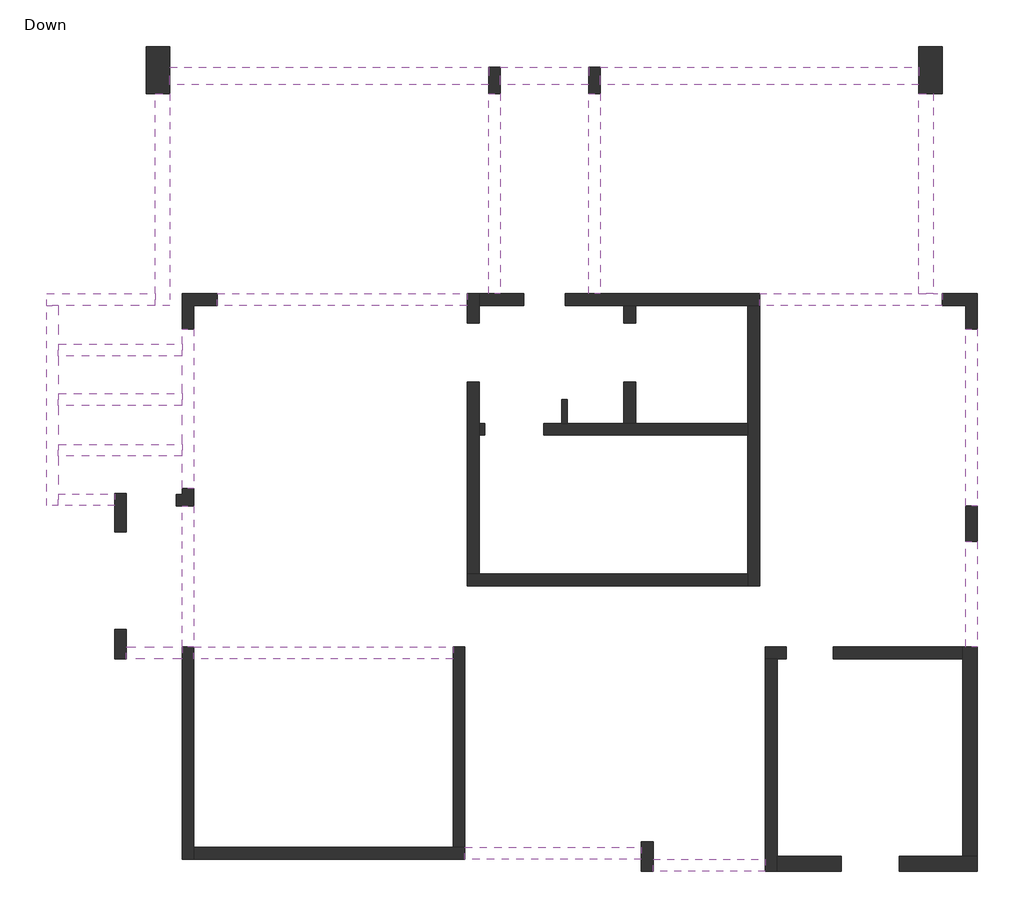
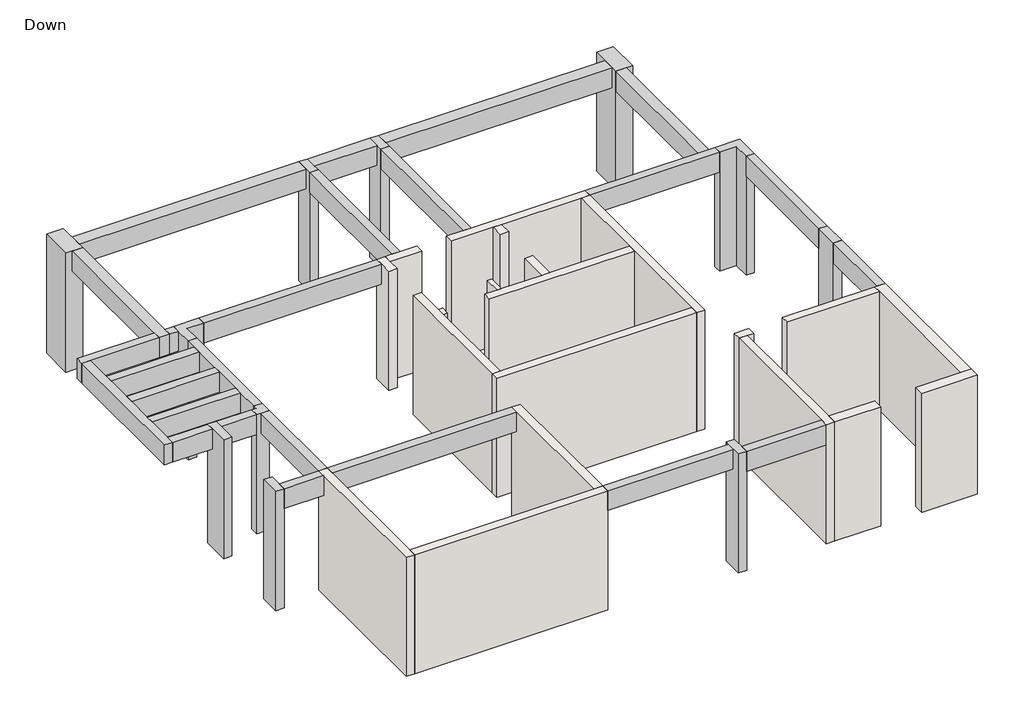
# One storey: 23 beams, 20 walls, 11 columns.
# Revit data of these elements (continued)
# Element 19 (IfcBeam, "Concrete Rectengular Beam : 25/50") (continued)
#   SOFiSTiK_AMG_Scheduled = yes
#   SOFiSTiK_AMG_Adjusted = yes
#   Structural Material = Concrete
#   Phase Created = New Construction
#   Materials on its faces: "Concrete"
# Element 20 (IfcBeam, "Concrete Rectengular Beam : 25/50")
#   Comments = ""
#   Mark = "B20"
#   SOFiSTiK_AMG_Comments = ""
#   SOFiSTiK_AMG_Scheduled = yes
#   SOFiSTiK_AMG_Adjusted = yes
#   Structural Material = Concrete
#   Phase Created = New Construction
#   Materials on its faces: "Concrete"
# Element 21 (IfcBeam, "Concrete Rectengular Beam : 30/50")
#   Comments = ""
#   Mark = "B21"
#   SOFiSTiK_AMG_Comments = ""
#   SOFiSTiK_AMG_Scheduled = yes
#   SOFiSTiK_AMG_Adjusted = yes
#   Structural Material = Concrete
#   Phase Created = New Construction
#   Materials on its faces: "Concrete"
# Element 22 (IfcBeam, "Concrete Rectengular Beam : 30/50")
#   Comments = ""
#   Mark = "B22"
#   SOFiSTiK_AMG_Comments = ""
#   SOFiSTiK_AMG_Scheduled = yes
#   SOFiSTiK_AMG_Adjusted = yes
#   Structural Material = Concrete
#   Phase Created = New Construction
#   Materials on its faces: "Concrete"
# Element 23 (IfcBeam, "Concrete Rectengular Beam : 30/50")
#   Comments = ""
#   Mark = "B23"
#   SOFiSTiK_AMG_Comments = ""
#   SOFiSTiK_AMG_Scheduled = yes
#   SOFiSTiK_AMG_Adjusted = yes
#   Structural Material = Concrete
#   Phase Created = New Construction
#   Materials on its faces: "Concrete"
# Element 24 (IfcColumn, "Concrete Rectengular Column : 20/45")
#   Comments = ""
#   Mark = "C1"
#   SOFiSTiK_AMG_Comments = ""
#   SOFiSTiK_AMG_Scheduled = yes
#   SOFiSTiK_AMG_Adjusted = yes
#   Structural Material = Concrete
#   Phase Created = New Construction
#   Materials on its faces: "Concrete"
# Element 25 (IfcColumn, "Concrete Rectengular Column : 20/45")
#   Comments = ""
#   Mark = "C2"
#   SOFiSTiK_AMG_Comments = ""
#   SOFiSTiK_AMG_Scheduled = yes
#   SOFiSTiK_AMG_Adjusted = yes
#   Structural Material = Concrete
#   Phase Created = New Construction
#   Materials on its faces: "Concrete"
# Element 26 (IfcColumn, "Concrete Rectengular Column : 20/50")
#   Comments = ""
#   Mark = "C3"
#   SOFiSTiK_AMG_Comments = ""
#   SOFiSTiK_AMG_Scheduled = yes
#   SOFiSTiK_AMG_Adjusted = yes
#   Structural Material = Concrete
#   Phase Created = New Construction
#   Materials on its faces: "Concrete"
# Element 27 (IfcColumn, "Concrete Rectengular Column : 20/50")
#   Comments = ""
#   Mark = "C4"
#   SOFiSTiK_AMG_Comments = ""
#   SOFiSTiK_AMG_Scheduled = yes
#   SOFiSTiK_AMG_Adjusted = yes
#   Structural Material = Concrete
#   Phase Created = New Construction
#   Materials on its faces: "Concrete"
# Element 28 (IfcColumn, "Concrete Rectengular Column : 20/60")
#   Comments = ""
#   Mark = "C5"
#   SOFiSTiK_AMG_Comments = ""
#   SOFiSTiK_AMG_Scheduled = yes
#   SOFiSTiK_AMG_Adjusted = yes
#   Structural Material = Concrete
#   Phase Created = New Construction
#   Materials on its faces: "Concrete"
# Element 29 (IfcColumn, "Concrete Rectengular Column : 20/65")
#   Comments = ""
#   Mark = "C6"
#   SOFiSTiK_AMG_Comments = ""
#   SOFiSTiK_AMG_Scheduled = yes
#   SOFiSTiK_AMG_Adjusted = yes
#   Structural Material = Concrete
#   Phase Created = New Construction
#   Materials on its faces: "Concrete"
# Element 30 (IfcColumn, "Concrete Rectengular Column : 40/80")
#   Comments = ""
#   Mark = "C7"
#   SOFiSTiK_AMG_Comments = ""
#   SOFiSTiK_AMG_Scheduled = yes
#   SOFiSTiK_AMG_Adjusted = yes
#   Structural Material = Concrete
#   Phase Created = New Construction
#   Materials on its faces: "Concrete"
# Element 31 (IfcColumn, "Concrete Rectengular Column : 40/80")
#   Comments = ""
#   Mark = "C8"
#   SOFiSTiK_AMG_Comments = ""
#   SOFiSTiK_AMG_Scheduled = yes
#   SOFiSTiK_AMG_Adjusted = yes
#   Structural Material = Concrete
#   Phase Created = New Construction
#   Materials on its faces: "Concrete"
# Element 32 (IfcColumn, "L Column : 30/30/20/20")
#   Comments = ""
#   Mark = "C9"
#   SOFiSTiK_AMG_Comments = ""
#   SOFiSTiK_AMG_Scheduled = yes
#   SOFiSTiK_AMG_Adjusted = yes
#   Structural Material = Concrete
#   Phase Created = New Construction
# Element 33 (IfcColumn, "L Column : 60/60/20/20")
#   Comments = ""
#   Mark = "C10"
#   SOFiSTiK_AMG_Comments = ""
#   SOFiSTiK_AMG_Scheduled = yes
#   SOFiSTiK_AMG_Adjusted = yes
#   Structural Material = Concrete
#   Phase Created = New Construction
# Element 34 (IfcColumn, "L Column : 60/60/20/20")
#   Comments = ""
#   Mark = "C11"
#   SOFiSTiK_AMG_Comments = ""
#   SOFiSTiK_AMG_Scheduled = yes
#   SOFiSTiK_AMG_Adjusted = yes
#   Structural Material = Concrete
#   Phase Created = New Construction
# Element 35 (IfcWall, "10")
#   Comments = ""
#   Mark = "W17"
#   SOFiSTiK_EdgeZones = "W17"
#   SOFiSTiK_AMG_Comments = "Too Narrow /"
#   Top Offset = 0 cm
#   Base Offset = 0 cm
#   wall height = 300 cm
#   SOFiSTiK_AMG_Scheduled = yes
#   SOFiSTiK_AMG_Adjusted = yes
#   Phase Created = New Construction
#   Base Constraint = Down
#   Top Constraint = Typical Floor
#   Materials on its faces: "Concrete"
# Element 36 (IfcWall, "20")
#   Comments = ""
#   Mark = "W1"
#   SOFiSTiK_EdgeZones = "W1"
#   SOFiSTiK_AMG_Comments = ""
#   Top Offset = 0 cm
#   Base Offset = 0 cm
#   wall height = 300 cm
#   SOFiSTiK_AMG_Scheduled = yes
#   SOFiSTiK_AMG_Adjusted = yes
#   Phase Created = New Construction
#   Base Constraint = Down
#   Top Constraint = Typical Floor
#   Materials on its faces: "Concrete"
# Element 37 (IfcWall, "20")
#   Comments = ""
#   Mark = "W2"
#   SOFiSTiK_EdgeZones = "W2"
#   SOFiSTiK_AMG_Comments = ""
#   Top Offset = 0 cm
#   Base Offset = 0 cm
#   wall height = 300 cm
#   SOFiSTiK_AMG_Scheduled = yes
#   SOFiSTiK_AMG_Adjusted = yes
#   Phase Created = New Construction
#   Base Constraint = Down
#   Top Constraint = Typical Floor
#   Materials on its faces: "Concrete"
# Element 38 (IfcWall, "20")
#   Comments = ""
#   Mark = "W3"
#   SOFiSTiK_EdgeZones = "W3"
#   SOFiSTiK_AMG_Comments = ""
#   Top Offset = 0 cm
#   Base Offset = 0 cm
#   wall height = 300 cm
#   SOFiSTiK_AMG_Scheduled = yes
#   SOFiSTiK_AMG_Adjusted = yes
#   Phase Created = New Construction
#   Base Constraint = Down
#   Top Constraint = Typical Floor
#   Materials on its faces: "Concrete"
# Element 39 (IfcWall, "20")
#   Comments = ""
#   Mark = "W4"
#   SOFiSTiK_EdgeZones = "W4"
#   SOFiSTiK_AMG_Comments = ""
#   Top Offset = 0 cm
#   Base Offset = 0 cm
#   wall height = 300 cm
#   SOFiSTiK_AMG_Scheduled = yes
#   SOFiSTiK_AMG_Adjusted = yes
#   Phase Created = New Construction
#   Base Constraint = Down
#   Top Constraint = Typical Floor
#   Materials on its faces: "Concrete"
# Element 40 (IfcWall, "20")
#   Comments = ""
#   Mark = "W5"
#   SOFiSTiK_EdgeZones = "W5"
#   SOFiSTiK_AMG_Comments = ""
#   Top Offset = 0 cm
#   Base Offset = 0 cm
#   wall height = 300 cm
#   SOFiSTiK_AMG_Scheduled = yes
#   SOFiSTiK_AMG_Adjusted = yes
#   Phase Created = New Construction
#   Base Constraint = Down
#   Top Constraint = Typical Floor
#   Materials on its faces: "Concrete"
# Element 41 (IfcWall, "20")
#   Comments = ""
#   Mark = "W6"
#   SOFiSTiK_EdgeZones = "W6"
#   SOFiSTiK_AMG_Comments = ""
#   Top Offset = 0 cm
#   Base Offset = 0 cm
#   wall height = 300 cm
#   SOFiSTiK_AMG_Scheduled = yes
#   SOFiSTiK_AMG_Adjusted = yes
#   Phase Created = New Construction
#   Base Constraint = Down
#   Top Constraint = Typical Floor
#   Materials on its faces: "Concrete"
# Element 42 (IfcWall, "20")
#   Comments = ""
#   Mark = "W7"
#   SOFiSTiK_EdgeZones = "W7"
#   SOFiSTiK_AMG_Comments = "Too Short /"
#   Top Offset = 0 cm
#   Base Offset = 0 cm
#   wall height = 300 cm
#   SOFiSTiK_AMG_Scheduled = yes
#   SOFiSTiK_AMG_Adjusted = yes
#   Phase Created = New Construction
#   Base Constraint = Down
#   Top Constraint = Typical Floor
#   Materials on its faces: "Concrete"
# Element 43 (IfcWall, "20")
#   Comments = ""
#   Mark = "W8"
#   SOFiSTiK_EdgeZones = "W8"
#   SOFiSTiK_AMG_Comments = ""
#   Top Offset = 0 cm
#   Base Offset = 0 cm
#   wall height = 300 cm
#   SOFiSTiK_AMG_Scheduled = yes
#   SOFiSTiK_AMG_Adjusted = yes
#   Phase Created = New Construction
#   Base Constraint = Down
#   Top Constraint = Typical Floor
#   Materials on its faces: "Concrete"
# Element 44 (IfcWall, "20")
#   Comments = ""
#   Mark = "W9"
#   SOFiSTiK_EdgeZones = "W9"
#   SOFiSTiK_AMG_Comments = ""
#   Top Offset = 0 cm
#   Base Offset = 0 cm
#   wall height = 300 cm
#   SOFiSTiK_AMG_Scheduled = yes
#   SOFiSTiK_AMG_Adjusted = yes
#   Phase Created = New Construction
#   Base Constraint = Down
#   Top Constraint = Typical Floor
#   Materials on its faces: "Concrete"
# Element 45 (IfcWall, "20")
#   Comments = ""
#   Mark = "W10"
#   SOFiSTiK_EdgeZones = "W10"
#   SOFiSTiK_AMG_Comments = ""
#   Top Offset = 0 cm
#   Base Offset = 0 cm
#   wall height = 300 cm
#   SOFiSTiK_AMG_Scheduled = yes
#   SOFiSTiK_AMG_Adjusted = yes
#   Phase Created = New Construction
#   Base Constraint = Down
#   Top Constraint = Typical Floor
#   Materials on its faces: "Concrete"
# Element 46 (IfcWall, "20")
#   Comments = ""
#   Mark = "W11"
#   SOFiSTiK_EdgeZones = "W11"
#   SOFiSTiK_AMG_Comments = ""
#   Top Offset = 0 cm
#   Base Offset = 0 cm
#   wall height = 300 cm
#   SOFiSTiK_AMG_Scheduled = yes
#   SOFiSTiK_AMG_Adjusted = yes
#   Phase Created = New Construction
#   Base Constraint = Down
#   Top Constraint = Typical Floor
#   Materials on its faces: "Concrete"
# Element 47 (IfcWall, "20")
#   Comments = ""
#   Mark = "W12"
#   SOFiSTiK_EdgeZones = "W12"
#   SOFiSTiK_AMG_Comments = ""
#   Top Offset = 0 cm
#   Base Offset = 0 cm
#   wall height = 300 cm
#   SOFiSTiK_AMG_Scheduled = yes
#   SOFiSTiK_AMG_Adjusted = yes
#   Phase Created = New Construction
#   Base Constraint = Down
#   Top Constraint = Typical Floor
#   Materials on its faces: "Concrete"
# Element 48 (IfcWall, "20")
#   Comments = ""
#   Mark = "W13"
#   SOFiSTiK_EdgeZones = "W13"
#   SOFiSTiK_AMG_Comments = ""
#   Top Offset = 0 cm
#   Base Offset = 0 cm
#   wall height = 300 cm
#   SOFiSTiK_AMG_Scheduled = yes
#   SOFiSTiK_AMG_Adjusted = yes
#   Phase Created = New Construction
#   Base Constraint = Down
#   Top Constraint = Typical Floor
#   Materials on its faces: "Concrete"
# Element 49 (IfcWall, "20")
#   Comments = ""
#   Mark = "W14"
#   SOFiSTiK_EdgeZones = "W14"
#   SOFiSTiK_AMG_Comments = ""
#   Top Offset = 0 cm
#   Base Offset = 0 cm
#   wall height = 300 cm
#   SOFiSTiK_AMG_Scheduled = yes
#   SOFiSTiK_AMG_Adjusted = yes
#   Phase Created = New Construction
#   Base Constraint = Down
#   Top Constraint = Typical Floor
#   Materials on its faces: "Concrete"
# Element 50 (IfcWall, "20")
#   Comments = ""
#   Mark = "W15"
#   SOFiSTiK_EdgeZones = "W15"
#   SOFiSTiK_AMG_Comments = ""
#   Top Offset = 0 cm
#   Base Offset = 0 cm
#   wall height = 300 cm
#   SOFiSTiK_AMG_Scheduled = yes
#   SOFiSTiK_AMG_Adjusted = yes
#   Phase Created = New Construction
#   Base Constraint = Down
#   Top Constraint = Typical Floor
#   Materials on its faces: "Concrete"
# Element 51 (IfcWall, "20")
#   Comments = ""
#   Mark = "W16"
#   SOFiSTiK_EdgeZones = "W16"
#   SOFiSTiK_AMG_Comments = ""
#   Top Offset = 0 cm
#   Base Offset = 0 cm
#   wall height = 300 cm
#   SOFiSTiK_AMG_Scheduled = yes
#   SOFiSTiK_AMG_Adjusted = yes
#   Phase Created = New Construction
#   Base Constraint = Down
#   Top Constraint = Typical Floor
#   Materials on its faces: "Concrete"
# Element 52 (IfcWall, "25")
#   Comments = ""
#   Mark = "W18"
#   SOFiSTiK_EdgeZones = "W18"
#   SOFiSTiK_AMG_Comments = ""
#   Top Offset = 0 cm
#   Base Offset = 0 cm
#   wall height = 300 cm
#   SOFiSTiK_AMG_Scheduled = yes
#   SOFiSTiK_AMG_Adjusted = yes
#   Phase Created = New Construction
#   Base Constraint = Down
#   Top Constraint = Typical Floor
#   Materials on its faces: "Concrete"
# Element 53 (IfcWall, "25")
#   Comments = ""
#   Mark = "W19"
#   SOFiSTiK_EdgeZones = "W19"
#   SOFiSTiK_AMG_Comments = ""
#   Top Offset = 0 cm
#   Base Offset = 0 cm
#   wall height = 300 cm
#   SOFiSTiK_AMG_Scheduled = yes
#   SOFiSTiK_AMG_Adjusted = yes
#   Phase Created = New Construction
#   Base Constraint = Down
#   Top Constraint = Typical Floor
#   Materials on its faces: "Concrete"
# Element 54 (IfcWall, "25")
#   Comments = ""
#   Mark = "W20"
#   SOFiSTiK_EdgeZones = "W20"
#   SOFiSTiK_AMG_Comments = ""
#   Top Offset = 0 cm
#   Base Offset = 0 cm
#   wall height = 300 cm
#   SOFiSTiK_AMG_Scheduled = yes
#   SOFiSTiK_AMG_Adjusted = yes
#   Phase Created = New Construction
#   Base Constraint = Down
#   Top Constraint = Typical Floor
#   Materials on its faces: "Concrete"
# Materials
#   "Concrete": class "Concrete", colour RGB 192 192 192, transparency 0, Keynote = "01000", Description = "Cast-in-place concrete", Cost = 0
#   "Concrete, Cast-in-Place gray": class "Concrete", colour RGB 192 192 192, transparency 0, Description = "Cast-in-place concrete", Cost = 0
